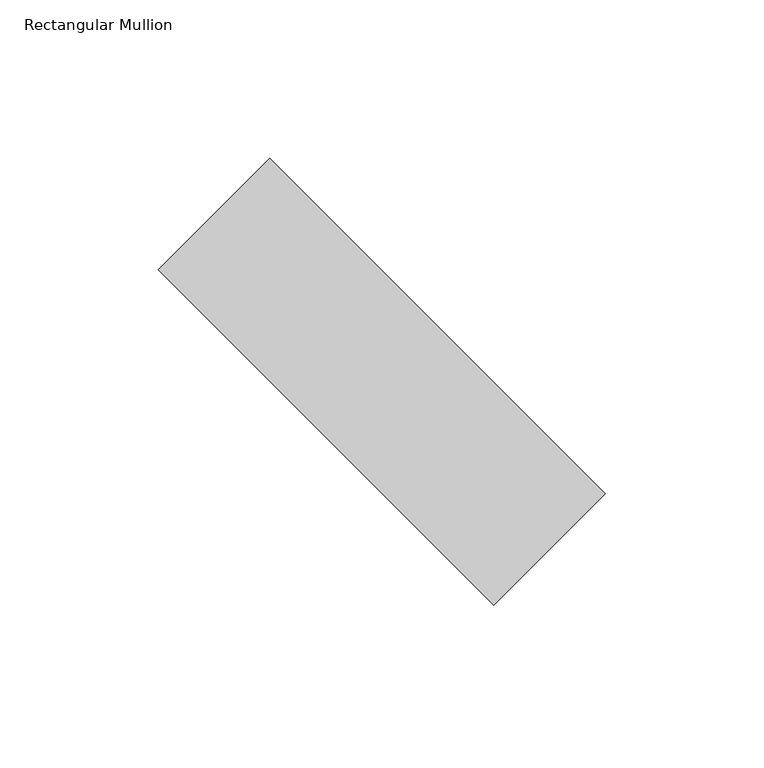
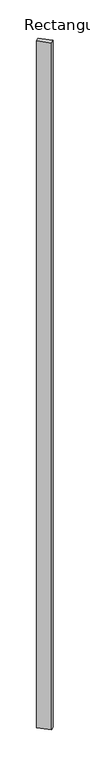
"""IFC4 building model written with IfcOpenShell, lengths in millimetres: member geometry, Rectangular Mullion : tilted mullions."""

from ifc_helpers import new_model, si_unit, frame, origin, place, context, project, spatial, polyline, outline, extrude, source, transform, mapped, element, save


def rectangular_mullion_5ffb7332(model_context):
    return source(origin(), model_context, "Body", "SweptSolid", [
        extrude(outline(polyline([(-35.3553391, 70.7106781), (70.7106781, -35.3553391), (35.3553391, -70.7106781), (-70.7106781, 35.3553391), (-35.3553391, 70.7106781)])), frame((0.0, 0.0, -7999.4864286), z_axis=(0.0, 0.0, 1.0), x_axis=(1.0, 0.0, 0.0)), (0.0, 0.0, 1.0), 7999.4864286),
    ])


if __name__ == "__main__":
    model = new_model("IFC4")
    model_context = context("Model", 3, world=origin())
    ifc_project = project(units=[si_unit("LENGTHUNIT", "METRE", prefix="MILLI")], contexts=[model_context])
    site = spatial("IfcSite", under=ifc_project)
    building = spatial("IfcBuilding", under=site)
    placement = place(None, origin())
    rectangular_mullion_shape = rectangular_mullion_5ffb7332(model_context)
    element("IfcMember", 1, ObjectType="Rectangular Mullion : tilted mullions", at=placement, inside=building, context=model_context, shape_type="MappedRepresentation", body=[
        mapped(rectangular_mullion_shape, transform((0.0, 0.0, 0.0), x_axis=(1.0, 0.0, 0.0), y_axis=(0.0, 1.0, 0.0), z_axis=(0.0, 0.0, 1.0))),
    ])
    save(model, "model.ifc")

# Revit data of these elements
# Type "Rectangular Mullion : tilted mullions"
#   built-in parameter 1007304 = 0.492126 (stored number, unit not read)
#   built-in parameter 1007301 = 0.082021 (stored number, unit not read)
#   built-in parameter 1007300 = 0.082021 (stored number, unit not read)
# Element 1 (IfcMember, "Rectangular Mullion : tilted mullions")
#   Materials on its faces: "Aluminum"
# Materials
#   "Aluminum": class "Metal", colour RGB 244 244 244, transparency 0, Description = "Aluminum 6061", Cost = 0
